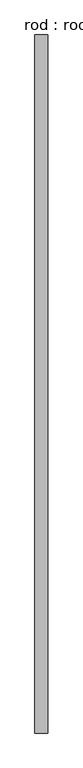
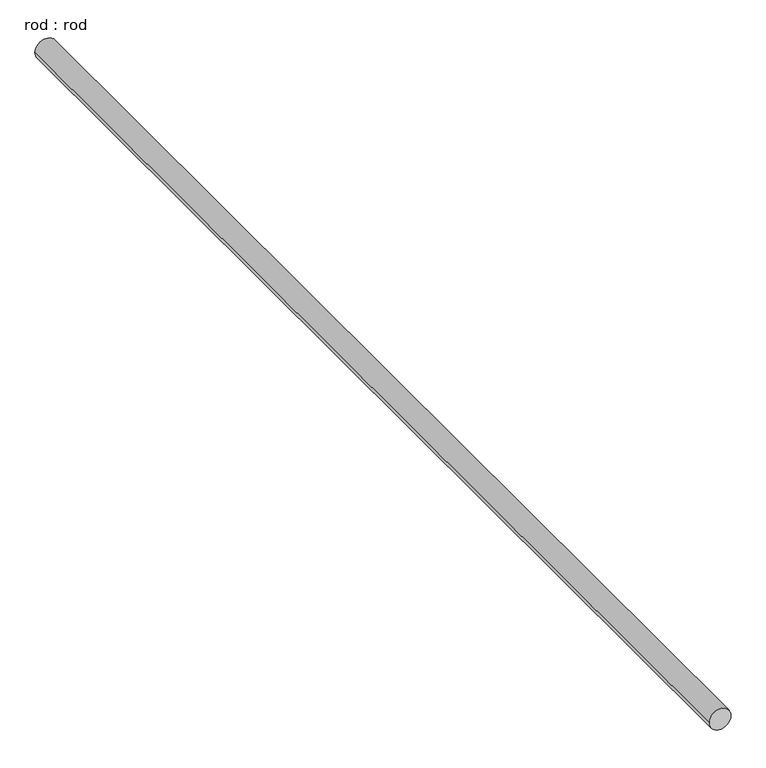
"""IFC4 building model written with IfcOpenShell, lengths in millimetres: proxy geometry, rod : rod."""

from ifc_helpers import new_model, si_unit, point, frame, frame_2d, origin, place, context, project, spatial, circle_curve, trimmed, segment, composite_curve, outline, extrude, source, transform, mapped, element, save


def rod_rod_667616aa(model_context):
    return source(origin(), model_context, "Body", "SweptSolid", [
        extrude(outline(composite_curve([segment(trimmed(circle_curve(frame_2d((0.0108462, 0.0)), 200.0), [point((0.0108462, 200.0))], [point((0.0108462, -200.0))], False, "CARTESIAN"), True, "CONTINUOUS"), segment(trimmed(circle_curve(frame_2d((0.0108462, 0.0)), 200.0), [point((0.0108462, -200.0))], [point((0.0108462, 200.0))], False, "CARTESIAN"), True, "CONTINUOUS")], self_intersect=False)), frame((0.0, -6592.8969871, 0.0), z_axis=(0.0, 1.0, 0.0), x_axis=(0.0, 0.0, 1.0)), (0.0, 0.0, 1.0), 21371.2512049),
    ])


if __name__ == "__main__":
    model = new_model("IFC4")
    model_context = context("Model", 3, world=origin())
    ifc_project = project(units=[si_unit("LENGTHUNIT", "METRE", prefix="MILLI")], contexts=[model_context])
    site = spatial("IfcSite", under=ifc_project)
    building = spatial("IfcBuilding", under=site)
    placement = place(None, origin())
    rod_rod_shape = rod_rod_667616aa(model_context)
    element("IfcBuildingElementProxy", 1, Name="rod : rod", ObjectType="rod : rod", at=placement, inside=building, context=model_context, shape_type="MappedRepresentation", body=[
        mapped(rod_rod_shape, transform((0.0, 0.0, 0.0), x_axis=(1.0, 0.0, 0.0), y_axis=(0.0, 1.0, 0.0), z_axis=(0.0, 0.0, 1.0))),
    ])
    save(model, "model.ifc")

# Revit data of these elements
# Type "rod : rod"
#   Default Elevation = 0
